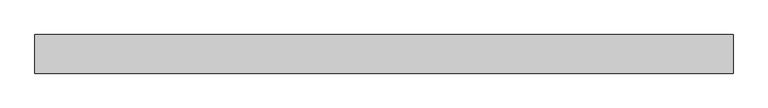
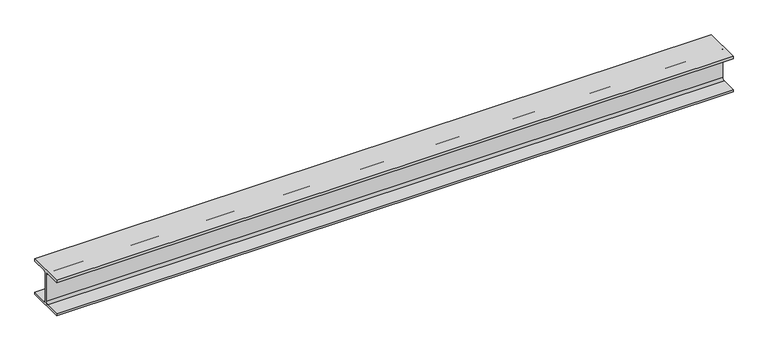
"""IFC4 building model written with IfcOpenShell, lengths in millimetres: beam geometry, 0912_Steel Framing_H-KSD3502 : H_SB_ASB_H-200x200x8x12."""

from ifc_helpers import new_model, si_unit, point, frame, frame_2d, origin, place, context, project, spatial, polyline, circle_curve, trimmed, segment, composite_curve, outline, extrude, source, transform, mapped, element, save


def beam_a92930dd(model_context):
    return source(origin(), model_context, "Body", "SweptSolid", [
        extrude(outline(composite_curve([segment(polyline([(100.0, -88.0), (100.0, -100.0), (-100.0, -100.0), (-100.0, -88.0), (-17.0, -88.0)]), True, "CONTINUOUS"), segment(trimmed(circle_curve(frame_2d((-17.0, -75.0)), 13.0), [point((-17.0, -88.0))], [point((-4.0, -75.0))], True, "CARTESIAN"), True, "CONTINUOUS"), segment(polyline([(-4.0, -75.0), (-4.0, 75.0)]), True, "CONTINUOUS"), segment(trimmed(circle_curve(frame_2d((-17.0, 75.0)), 13.0), [point((-4.0, 75.0))], [point((-17.0, 88.0))], True, "CARTESIAN"), True, "CONTINUOUS"), segment(polyline([(-17.0, 88.0), (-100.0, 88.0), (-100.0, 100.0), (100.0, 100.0), (100.0, 88.0), (17.0, 88.0)]), True, "CONTINUOUS"), segment(trimmed(circle_curve(frame_2d((17.0, 75.0)), 13.0), [point((17.0, 88.0))], [point((4.0, 75.0))], True, "CARTESIAN"), True, "CONTINUOUS"), segment(polyline([(4.0, 75.0), (4.0, -75.0)]), True, "CONTINUOUS"), segment(trimmed(circle_curve(frame_2d((17.0, -75.0)), 13.0), [point((4.0, -75.0))], [point((17.0, -88.0))], True, "CARTESIAN"), True, "CONTINUOUS"), segment(polyline([(17.0, -88.0), (100.0, -88.0)]), True, "CONTINUOUS")], self_intersect=False)), frame((-1666.7080909, 0.0, 0.0), z_axis=(1.0, 0.0, 0.0), x_axis=(0.0, 1.0, 0.0)), (0.0, 0.0, 1.0), 3611.1914237),
    ])


if __name__ == "__main__":
    model = new_model("IFC4")
    model_context = context("Model", 3, world=origin())
    ifc_project = project(units=[si_unit("LENGTHUNIT", "METRE", prefix="MILLI")], contexts=[model_context])
    site = spatial("IfcSite", under=ifc_project)
    building = spatial("IfcBuilding", under=site)
    placement = place(None, origin())
    beam_shape = beam_a92930dd(model_context)
    element("IfcBeam", 1, ObjectType="0912_Steel Framing_H-KSD3502 : H_SB_ASB_H-200x200x8x12", at=placement, inside=building, context=model_context, shape_type="MappedRepresentation", body=[
        mapped(beam_shape, transform((0.0, 0.0, 0.0), x_axis=(1.0, 0.0, 0.0), y_axis=(0.0, 1.0, 0.0), z_axis=(0.0, 0.0, 1.0))),
    ])
    save(model, "model.ifc")

# Revit data of these elements
# Type "0912_Steel Framing_H-KSD3502 : H_SB_ASB_H-200x200x8x12"
#   H_WM Code_1 = "S01AA002-00001 | Main Steel Structure Fabrication Work | Shelter/Building | Medium Steel - Standard (90KG/M>Weight≥30KG/M) | Material: (   )"
#   H_WM Code_2 = "S03AA028-00001 | Main Steel Structure Erection Work | Shelter/Building | Medium Steel (90KG/M>Weight≥30KG/M) | Material: (   )"
#   H_WM Code_3 = "S01AA010-00001 | Main Steel Structure Fabrication Work | Shelter/Building | Steel Painting/Coating | for Non-Fireproofed Steel Surface, Surface Preparation, Primer, Second & Final Coat | Material: (   )"
#   H_Q'ty Cal Type Tag = "SB-Q2"
#   Width = 20.0 cm
#   Web Thickness = 0.8 cm
#   Web Fillet = 1.3 cm
#   Warping Constant = 141000.0 cm⁶
#   W = 0
#   Torsional Moment of Inertia = 26.2485 cm⁴
#   Section Area = 63.53 cm²
#   Plastic Modulus weak axis = 244.0 cm³
#   Plastic Modulus strong axis = 525.0 cm³
#   Perimeter = 1.16 m²/m
#   Nominal Weight = 49.90 kgf/m
#   Moment of Inertia weak axis = 1600.00 cm⁴
#   Moment of Inertia strong axis = 4720.00 cm⁴
#   Height = 20.0 cm
#   Flange Thickness = 1.2 cm
#   Elastic Modulus weak axis = 160.0 cm³
#   Elastic Modulus strong axis = 472.0 cm³
#   Centroid Vertical = 10.0 cm
#   Centroid Horizontal = 10.0 cm
#   Ix = 47200000
#   Length [instance default] = 1.5240 m
#   Zx = 525000
#   b = 0.2000 m
#   h = 0.2000 m
#   r = 0.0130 m
#   s = 0.0080 m
#   t = 0.0120 m
#   A = 0.006353 m²
#   Structural Material [instance default] = Steel, 45-345
#   Assembly Code = ""
# Element 1 (IfcBeam, "0912_Steel Framing_H-KSD3502 : H_SB_ASB_H-200x200x8x12")
#   Structural Material = none
# Materials
#   "Steel, 45-345": class "Metal", colour RGB 189 187 185, transparency 0, Description = "Steel 345 MPa", Cost = 0
